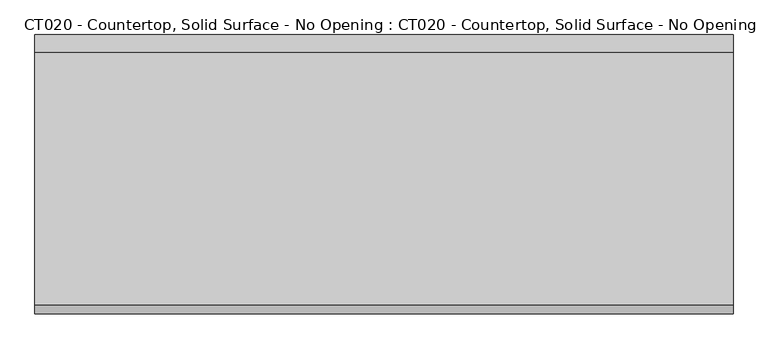
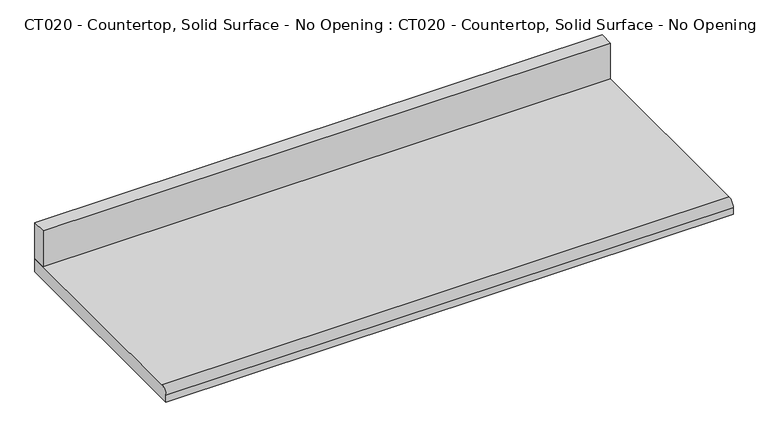
"""IFC4 building model written with IfcOpenShell, lengths in millimetres: proxy geometry, CT020 - Countertop, Solid Surface - No Opening : CT020 - Countertop, Solid Surface - No Opening."""

import ifcopenshell
import ifcopenshell.guid

model = None  # the IFC model being written
_history = None  # IfcOwnerHistory: only IFC2X3 demands one
_inside = {}  # id of a spatial element -> (the spatial element, [elements in it])
_under = {}  # id of a project, library or spatial element -> (it, [spatial elements below it])
_declared = {}  # id of a project -> (the project, [libraries it declares])
_typed = {}  # id of a type object -> (the type object, [elements of that type])
_made_of = {}  # id of a material, layer set ... -> (it, [elements and type objects made of it])


def new_model(schema):
    """Start an empty IFC model of exactly this schema.

    Asked for "IFC4X3", IfcOpenShell would pick the latest addendum, in which some entities
    have other attributes; the version numbers below select the first issue.
    IFC2X3 requires an IfcOwnerHistory on every rooted entity: one is made here for all.
    """
    global model, _history
    if schema == "IFC4X3":
        model = ifcopenshell.file(schema_version=(4, 3, 0, 0))
    else:
        model = ifcopenshell.file(schema=schema)
    _inside.clear()
    _under.clear()
    _declared.clear()
    _typed.clear()
    _made_of.clear()
    _history = None
    if model.schema == "IFC2X3":
        org = make("IfcOrganization", Name="unknown")
        user = make(
            "IfcPersonAndOrganization",
            ThePerson=make("IfcPerson", FamilyName="unknown"),
            TheOrganization=org,
        )
        app = make(
            "IfcApplication",
            ApplicationDeveloper=org,
            Version="unknown",
            ApplicationFullName="unknown",
            ApplicationIdentifier="unknown",
        )
        _history = make(
            "IfcOwnerHistory",
            OwningUser=user,
            OwningApplication=app,
            ChangeAction="ADDED",
            CreationDate=0,
        )
    return model


def make(cls, **values):
    """One entity of the class cls with the attributes given. An attribute that is None is left unset."""
    return model.create_entity(
        cls, **{name: value for name, value in values.items() if value is not None}
    )


def rooted(cls, **values):
    """An entity with a GlobalId (a new one), such as an element, a storey or a relation."""
    return make(cls, GlobalId=ifcopenshell.guid.new(), OwnerHistory=_history, **values)


def si_unit(unit_type, name, prefix=None):
    """IfcSIUnit, for example si_unit("LENGTHUNIT", "METRE", prefix="MILLI")."""
    return make("IfcSIUnit", UnitType=unit_type, Prefix=prefix, Name=name)


def assignment(units):
    """IfcUnitAssignment: the units of a project."""
    return None if units is None else make("IfcUnitAssignment", Units=units)


def point(xyz):
    """IfcCartesianPoint."""
    return None if xyz is None else make("IfcCartesianPoint", Coordinates=xyz)


def direction(xyz):
    """IfcDirection."""
    return None if xyz is None else make("IfcDirection", DirectionRatios=xyz)


def frame(location, z_axis=None, x_axis=None):
    """IfcAxis2Placement3D, a coordinate frame: its origin and axes. An axis left out is left unset."""
    return make(
        "IfcAxis2Placement3D",
        Location=point(location),
        Axis=direction(z_axis),
        RefDirection=direction(x_axis),
    )


def frame_2d(location, x_axis=None):
    """IfcAxis2Placement2D, a coordinate frame in the plane: its origin and x axis."""
    return make(
        "IfcAxis2Placement2D", Location=point(location), RefDirection=direction(x_axis)
    )


def origin():
    """The frame at (0, 0, 0) with its axes left unset."""
    return frame((0.0, 0.0, 0.0))


def place(relative_to, where):
    """IfcLocalPlacement: puts the frame where relative to a parent placement (None: the world)."""
    return make(
        "IfcLocalPlacement", PlacementRelTo=relative_to, RelativePlacement=where
    )


def context(
    kind, dimensions, precision=None, world=None, true_north=None, identifier=None
):
    """IfcGeometricRepresentationContext, for example the 3D "Model" context."""
    return make(
        "IfcGeometricRepresentationContext",
        ContextIdentifier=identifier,
        ContextType=kind,
        CoordinateSpaceDimension=dimensions,
        Precision=precision,
        WorldCoordinateSystem=world,
        TrueNorth=true_north,
    )


def project(units=None, contexts=None):
    """IfcProject with its units and contexts."""
    return rooted(
        "IfcProject",
        Name="project",
        RepresentationContexts=contexts,
        UnitsInContext=assignment(units),
    )


def spatial(cls, under=None, at=None, **own):
    """A site, building, storey or space (cls), placed at a placement, below another one or the project."""
    s = rooted(cls, ObjectPlacement=at, **own)
    if under is not None:
        _under.setdefault(under.id(), (under, []))[1].append(s)
    return s


def polyline(points):
    """IfcPolyline through the points."""
    return make("IfcPolyline", Points=[point(p) for p in points])


def circle_curve(where, radius):
    """IfcCircle in the frame where."""
    return make("IfcCircle", Position=where, Radius=radius)


def trimmed(basis, trim1, trim2, sense, master):
    """IfcTrimmedCurve: the piece of a basis curve between two trims."""
    return make(
        "IfcTrimmedCurve",
        BasisCurve=basis,
        Trim1=trim1,
        Trim2=trim2,
        SenseAgreement=sense,
        MasterRepresentation=master,
    )


def segment(curve, same_sense, transition):
    """IfcCompositeCurveSegment."""
    return make(
        "IfcCompositeCurveSegment",
        Transition=transition,
        SameSense=same_sense,
        ParentCurve=curve,
    )


def composite_curve(segments, self_intersect=None):
    """IfcCompositeCurve: segments joined end to end."""
    return make("IfcCompositeCurve", Segments=segments, SelfIntersect=self_intersect)


def outline(outer, holes=None, kind="AREA"):
    """IfcArbitraryClosedProfileDef: a profile drawn as a closed curve; with holes, ...WithVoids."""
    if holes is None:
        return make("IfcArbitraryClosedProfileDef", ProfileType=kind, OuterCurve=outer)
    return make(
        "IfcArbitraryProfileDefWithVoids",
        ProfileType=kind,
        OuterCurve=outer,
        InnerCurves=holes,
    )


def extrude(swept, where, along, depth):
    """IfcExtrudedAreaSolid: the profile swept, set in the frame where, extruded along a direction by depth."""
    return make(
        "IfcExtrudedAreaSolid",
        SweptArea=swept,
        Position=where,
        ExtrudedDirection=direction(along),
        Depth=depth,
    )


def shape(context_of_items, identifier, shape_type, items):
    """IfcShapeRepresentation: the items that make up one representation, for example the "Body"."""
    return make(
        "IfcShapeRepresentation",
        ContextOfItems=context_of_items,
        RepresentationIdentifier=identifier,
        RepresentationType=shape_type,
        Items=items,
    )


def source(mapping_origin, context_of_items, identifier, shape_type, items):
    """IfcRepresentationMap: a shape defined once, which mapped items show again and again."""
    return make(
        "IfcRepresentationMap",
        MappingOrigin=mapping_origin,
        MappedRepresentation=shape(context_of_items, identifier, shape_type, items),
    )


def transform(
    local_origin,
    x_axis=None,
    y_axis=None,
    z_axis=None,
    scale=None,
    scale2=None,
    scale3=None,
    uniform=True,
):
    """IfcCartesianTransformationOperator3D, or its non-uniform kind. x_axis, y_axis, z_axis: its Axis1, 2, 3."""
    if uniform:
        return make(
            "IfcCartesianTransformationOperator3D",
            Axis1=direction(x_axis),
            Axis2=direction(y_axis),
            LocalOrigin=point(local_origin),
            Scale=scale,
            Axis3=direction(z_axis),
        )
    return make(
        "IfcCartesianTransformationOperator3DnonUniform",
        Axis1=direction(x_axis),
        Axis2=direction(y_axis),
        LocalOrigin=point(local_origin),
        Scale=scale,
        Axis3=direction(z_axis),
        Scale2=scale2,
        Scale3=scale3,
    )


def mapped(mapping_source, mapping_target):
    """IfcMappedItem: shows the shape of a source again, moved by a transform."""
    return make(
        "IfcMappedItem", MappingSource=mapping_source, MappingTarget=mapping_target
    )


def made_of(thing, what):
    """Note that an element or type object is made of a material, layer set ...; save() writes the relation."""
    if what is not None:
        _made_of.setdefault(what.id(), (what, []))[1].append(thing)
    return thing


def element(
    cls,
    number,
    at=None,
    inside=None,
    cuts=None,
    type_object=None,
    material=None,
    context=None,
    identifier="Body",
    shape_type=None,
    held_by="IfcProductDefinitionShape",
    body=None,
    shapes=None,
    **own,
):
    """One element of the class cls, such as IfcWall. Its Tag is "e" and its number.

    at: its placement. inside: the storey or other place that contains it. cuts: it is an
    opening in that element (IfcRelVoidsElement). A single representation is given by context,
    identifier, shape_type and body (its items); several are given by shapes. held_by: the class
    of the entity that holds the representations. save() writes the other relations.
    """
    e = rooted(cls, Tag="e%d" % number, ObjectPlacement=at, **own)
    if body is not None:
        shapes = [shape(context, identifier, shape_type, body)]
    if shapes is not None:
        e.Representation = make(held_by, Representations=shapes)
    if inside is not None:
        _inside.setdefault(inside.id(), (inside, []))[1].append(e)
    if cuts is not None:
        rooted(
            "IfcRelVoidsElement", RelatingBuildingElement=cuts, RelatedOpeningElement=e
        )
    if type_object is not None:
        _typed.setdefault(type_object.id(), (type_object, []))[1].append(e)
    return made_of(e, material)


def aggregate(whole, parts):
    """IfcRelAggregates: a whole, such as a stair, and the parts it consists of."""
    return rooted("IfcRelAggregates", RelatingObject=whole, RelatedObjects=parts)


def save(model, path):
    """Write the relations noted so far, then the file.

    IfcRelAggregates (storeys below a building ...), IfcRelContainedInSpatialStructure (elements
    in a storey), IfcRelDefinesByType, IfcRelAssociatesMaterial and IfcRelDeclares: one each for
    every whole, place, type object, material and project.
    """
    for whole, parts in _under.values():
        aggregate(whole, parts)
    for where, things in _inside.values():
        rooted(
            "IfcRelContainedInSpatialStructure",
            RelatedElements=things,
            RelatingStructure=where,
        )
    for kind, things in _typed.values():
        rooted("IfcRelDefinesByType", RelatedObjects=things, RelatingType=kind)
    for what, things in _made_of.values():
        rooted("IfcRelAssociatesMaterial", RelatedObjects=things, RelatingMaterial=what)
    for by, libraries in _declared.values():
        rooted("IfcRelDeclares", RelatingContext=by, RelatedDefinitions=libraries)
    model.write(path)


def ct020_countertop_solid_surface_no_opening_ct020_countertop_9887f39e(model_context):
    return source(origin(), model_context, "Body", "SweptSolid", [
        extrude(outline(polyline([(-762.0, 266.7), (-762.0, 304.8), (762.0, 304.8), (762.0, 266.7), (-762.0, 266.7)])), frame((0.0, 0.0, 863.6), z_axis=(0.0, 0.0, 1.0), x_axis=(1.0, 0.0, 0.0)), (0.0, 0.0, 1.0), 101.6),
        extrude(outline(composite_curve([segment(polyline([(-285.75, 863.6), (304.8, 863.6), (304.8, 825.5), (-304.8, 825.5), (-304.8, 844.55)]), True, "CONTINUOUS"), segment(trimmed(circle_curve(frame_2d((-285.75, 844.55)), 19.05), [point((-304.8, 844.55))], [point((-285.75, 863.6))], False, "CARTESIAN"), True, "CONTINUOUS")], self_intersect=False)), frame((-762.0, 0.0, 0.0), z_axis=(1.0, 0.0, 0.0), x_axis=(0.0, 1.0, 0.0)), (0.0, 0.0, 1.0), 1524.0),
    ])


if __name__ == "__main__":
    model = new_model("IFC4")
    model_context = context("Model", 3, world=origin())
    ifc_project = project(units=[si_unit("LENGTHUNIT", "METRE", prefix="MILLI")], contexts=[model_context])
    site = spatial("IfcSite", under=ifc_project)
    building = spatial("IfcBuilding", under=site)
    placement = place(None, origin())
    ct020_countertop_solid_surface_no_opening_ct020_countertop_shape = ct020_countertop_solid_surface_no_opening_ct020_countertop_9887f39e(model_context)
    element("IfcBuildingElementProxy", 1, Name="CT020 - Countertop, Solid Surface - No Opening : CT020 - Countertop, Solid Surface - No Opening", ObjectType="CT020 - Countertop, Solid Surface - No Opening : CT020 - Countertop, Solid Surface - No Opening", at=placement, inside=building, context=model_context, shape_type="MappedRepresentation", body=[
        mapped(ct020_countertop_solid_surface_no_opening_ct020_countertop_shape, transform((0.0, 0.0, 0.0), x_axis=(1.0, 0.0, 0.0), y_axis=(0.0, 1.0, 0.0), z_axis=(0.0, 0.0, 1.0))),
    ])
    save(model, "model.ifc")

# Revit data of these elements
# Type "CT020 - Countertop, Solid Surface - No Opening : CT020 - Countertop, Solid Surface - No Opening"
#   Watts2 = "0"
#   Watts1 = "0"
#   Unit_Issue = "LF"
#   UTIL_6_Misc = "-"
#   UTIL_5_NonMedGas = "-"
#   UTIL_4_MiscGas = "-"
#   UTIL_3_MedGas = "-"
#   UTIL_2_Elec = "-"
#   UTIL_1_WaterDrain = "-"
#   Nomenclature = "Countertop, Solid Surface"
#   NSN = ""
#   Location [instance default] = ""
#   JSN = "CT020"
#   Fund_Source_VA = "-"
#   Fund_Source_Navy = "-"
#   Fund_Source_Army = "-"
#   Fund_Source_AF = "-"
#   ELEC_Volts2 = "0"
#   ELEC_Volts1 = "0"
#   ELEC_Phase2 = "0"
#   ELEC_Phase1 = "0"
#   ELEC_HertzSwitch = "0"
#   ELEC_HertzDependent = "0"
#   ELEC_Hertz = "0"
#   ELEC_Amps2 = "0"
#   ELEC_Amps1 = "0"
#   DetailDescription = ""
#   CAT_VA = "A"
#   CAT_Navy = "A"
#   CAT_IHS = "-"
#   CAT_Army = "A"
#   CAT_AF = "A"
#   BTUperhour = "0"
#   Weight_IP = 14
#   DIM_Width_IP = 1' - 0"
#   DIM_Height_IP = 0' - 1"
#   DIM_Depth_IP = 2' - 0"
#   CustomLength [instance default] = 6' - 0"
#   Assembly Code = ""
# Element 1 (IfcBuildingElementProxy, "CT020 - Countertop, Solid Surface - No Opening : CT020 - Countertop, Solid Surface - No Opening")
#   Location = "DNXS1"
#   CustomLength = 5' - 0"
#   Materials on its faces: "CounterTopFinish"
# Materials
#   "CounterTopFinish": class "Unassigned", colour RGB 139 121 96, transparency 0
